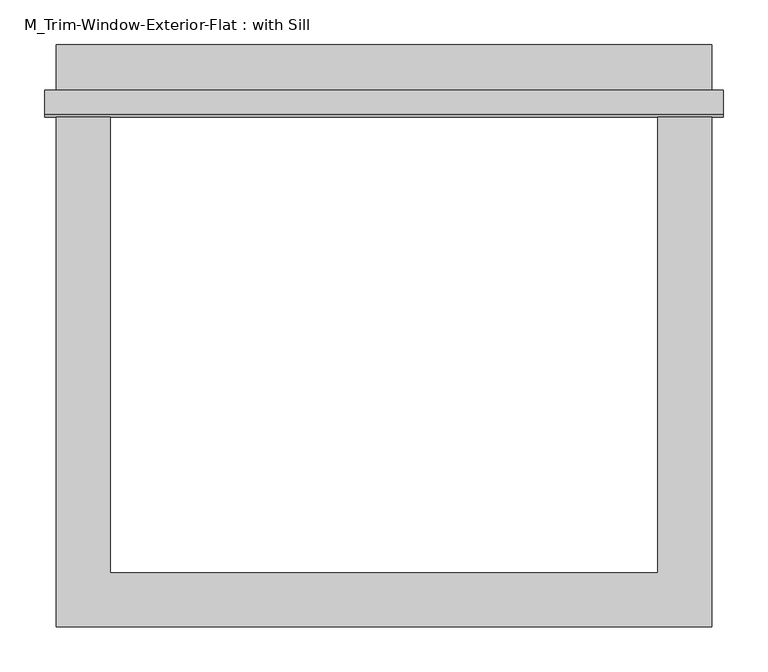
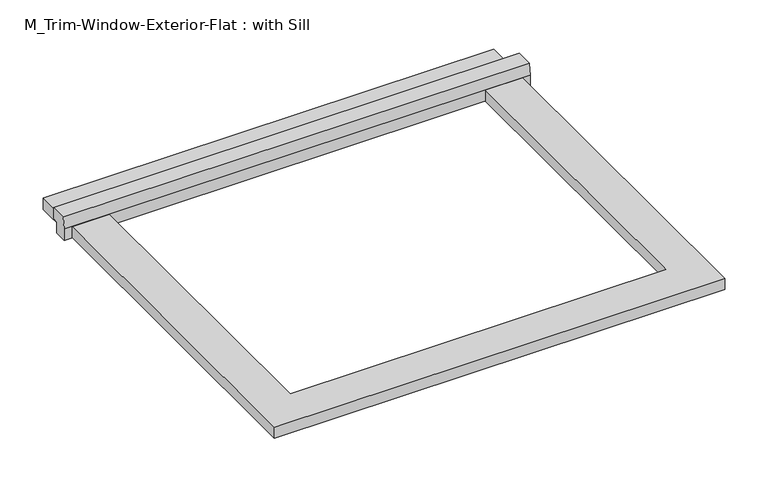
"""IFC4 building model written with IfcOpenShell, lengths in millimetres: proxy geometry, M_Trim-Window-Exterior-Flat : with Sill."""

from ifc_helpers import new_model, si_unit, frame, origin, origin_with_axes, place, context, project, spatial, polyline, outline, extrude, source, transform, mapped, element, save


def m_trim_window_exterior_flat_with_sill_c63465ee(model_context):
    return source(origin(), model_context, "Body", "SweptSolid", [
        extrude(outline(polyline([(364.8, 528.4323709), (-364.8, 528.4323709), (-364.8, 588.4323709), (364.8, 588.4323709), (364.8, 528.4323709)])), origin_with_axes(), (0.0, 0.0, 1.0), 19.05),
        extrude(outline(polyline([(538.0, 38.1), (538.0, 19.05), (528.4323709, 19.05), (528.4323709, 0.0), (508.0, 0.0), (508.0, 19.05), (510.4580645, 38.1), (538.0, 38.1)])), frame((-377.5, 0.0, 0.0), z_axis=(1.0, 0.0, 0.0), x_axis=(0.0, 1.0, 0.0)), (0.0, 0.0, 1.0), 755.0),
        extrude(outline(polyline([(-364.8, -60.0), (-364.8, 508.0), (-304.8, 508.0), (-304.8, 0.0), (304.8, 0.0), (304.8, 508.0), (364.8, 508.0), (364.8, -60.0), (-364.8, -60.0)])), origin_with_axes(), (0.0, 0.0, 1.0), 19.05),
    ])


if __name__ == "__main__":
    model = new_model("IFC4")
    model_context = context("Model", 3, world=origin())
    ifc_project = project(units=[si_unit("LENGTHUNIT", "METRE", prefix="MILLI")], contexts=[model_context])
    site = spatial("IfcSite", under=ifc_project)
    building = spatial("IfcBuilding", under=site)
    placement = place(None, origin())
    m_trim_window_exterior_flat_with_sill_shape = m_trim_window_exterior_flat_with_sill_c63465ee(model_context)
    element("IfcBuildingElementProxy", 1, Name="M_Trim-Window-Exterior-Flat : with Sill", ObjectType="M_Trim-Window-Exterior-Flat : with Sill", at=placement, inside=building, context=model_context, shape_type="MappedRepresentation", body=[
        mapped(m_trim_window_exterior_flat_with_sill_shape, transform((0.0, 0.0, 0.0), x_axis=(1.0, 0.0, 0.0), y_axis=(0.0, 1.0, 0.0), z_axis=(0.0, 0.0, 1.0))),
    ])
    save(model, "model.ifc")

# Revit data of these elements
# Type "M_Trim-Window-Exterior-Flat : with Sill"
#   Trim Width = 0' - 2.3622"
#   Trim Thickness_Picture Frame = 0' - 1.1811"
#   Trim Thickness_with Sill = 0' - 0 3/4"
#   Sill Thickness = 0' - 1.1811"
#   Opening Width [instance default] = 1' - 11.62205"
#   Opening Height [instance default] = 2' - 11.43307"
#   Default Elevation = 3' - 11.24409"
#   Sill = yes
#   Picture Frame = no
#   Trim Material [instance default] = none
# Element 1 (IfcBuildingElementProxy, "M_Trim-Window-Exterior-Flat : with Sill")
#   Opening Width = 2' - 0"
#   Opening Height = 1' - 8"
#   Trim Material = Clad - White
#   Materials on its faces: "Clad - White"
# Materials
#   "Clad - White": class "Wood", colour RGB 242 242 238, transparency 0, Cost = 0
